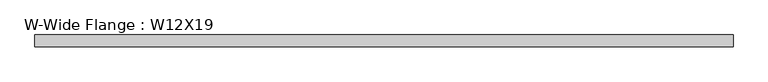
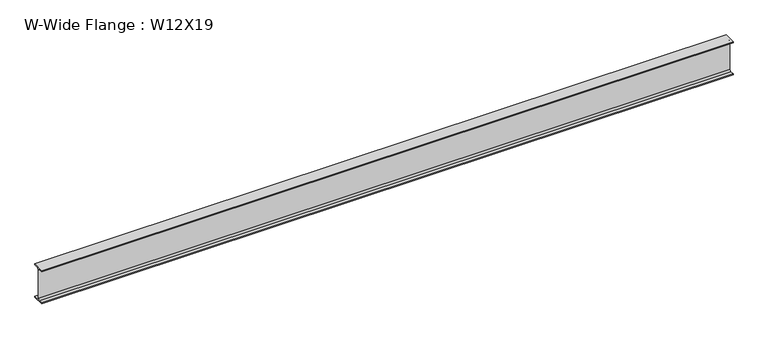
"""IFC4 building model written with IfcOpenShell, lengths in millimetres: beam geometry, W-Wide Flange : W12X19."""

from ifc_helpers import new_model, si_unit, point, frame, frame_2d, origin, place, context, project, spatial, polyline, circle_curve, trimmed, segment, composite_curve, outline, extrude, source, transform, mapped, element, save


def w_wide_flange_w12x19_3ac24698(model_context):
    return source(origin(), model_context, "Body", "SweptSolid", [
        extrude(outline(composite_curve([segment(polyline([(50.927, -146.05), (50.927, -154.94), (-50.927, -154.94), (-50.927, -146.05), (-16.3195, -146.05)]), True, "CONTINUOUS"), segment(trimmed(circle_curve(frame_2d((-16.3195, -132.715)), 13.335), [point((-16.3195, -146.05))], [point((-2.9845, -132.715))], True, "CARTESIAN"), True, "CONTINUOUS"), segment(polyline([(-2.9845, -132.715), (-2.9845, 132.715)]), True, "CONTINUOUS"), segment(trimmed(circle_curve(frame_2d((-16.3195, 132.715)), 13.335), [point((-2.9845, 132.715))], [point((-16.3195, 146.05))], True, "CARTESIAN"), True, "CONTINUOUS"), segment(polyline([(-16.3195, 146.05), (-50.927, 146.05), (-50.927, 154.94), (50.927, 154.94), (50.927, 146.05), (16.3195, 146.05)]), True, "CONTINUOUS"), segment(trimmed(circle_curve(frame_2d((16.3195, 132.715)), 13.335), [point((16.3195, 146.05))], [point((2.9845, 132.715))], True, "CARTESIAN"), True, "CONTINUOUS"), segment(polyline([(2.9845, 132.715), (2.9845, -132.715)]), True, "CONTINUOUS"), segment(trimmed(circle_curve(frame_2d((16.3195, -132.715)), 13.335), [point((2.9845, -132.715))], [point((16.3195, -146.05))], True, "CARTESIAN"), True, "CONTINUOUS"), segment(polyline([(16.3195, -146.05), (50.927, -146.05)]), True, "CONTINUOUS")], self_intersect=False)), frame((-3035.3, 0.0, 0.0), z_axis=(1.0, 0.0, 0.0), x_axis=(0.0, 1.0, 0.0)), (0.0, 0.0, 1.0), 6070.6),
    ])


if __name__ == "__main__":
    model = new_model("IFC4")
    model_context = context("Model", 3, world=origin())
    ifc_project = project(units=[si_unit("LENGTHUNIT", "METRE", prefix="MILLI")], contexts=[model_context])
    site = spatial("IfcSite", under=ifc_project)
    building = spatial("IfcBuilding", under=site)
    placement = place(None, origin())
    w_wide_flange_w12x19_shape = w_wide_flange_w12x19_3ac24698(model_context)
    element("IfcBeam", 1, ObjectType="W-Wide Flange : W12X19", at=placement, inside=building, context=model_context, shape_type="MappedRepresentation", body=[
        mapped(w_wide_flange_w12x19_shape, transform((0.0, 0.0, 0.0), x_axis=(1.0, 0.0, 0.0), y_axis=(0.0, 1.0, 0.0), z_axis=(0.0, 0.0, 1.0))),
    ])
    save(model, "model.ifc")

# Revit data of these elements
# Type "W-Wide Flange : W12X19"
#   Assembly Code = "B10"
#   W = 19
#   Length [instance default] = 5' - 0"
#   bf = 0' - 4.01"
#   d = 1' - 0.2"
#   k = 0' - 0 7/8"
#   k2 = 0' - 0.525"
#   tf = 0' - 0.35"
#   tw = 0' - 0.235"
#   A = 0.0386806 SF
#   Structural Material [instance default] = Steel ASTM A992
# Element 1 (IfcBeam, "W-Wide Flange : W12X19")
#   Materials on its faces: "Steel ASTM A992"
# Materials
#   "Steel ASTM A992": class "Metal", colour RGB 199 199 199, transparency 0, Description = "Structural steel 50ksi", Cost = 0
